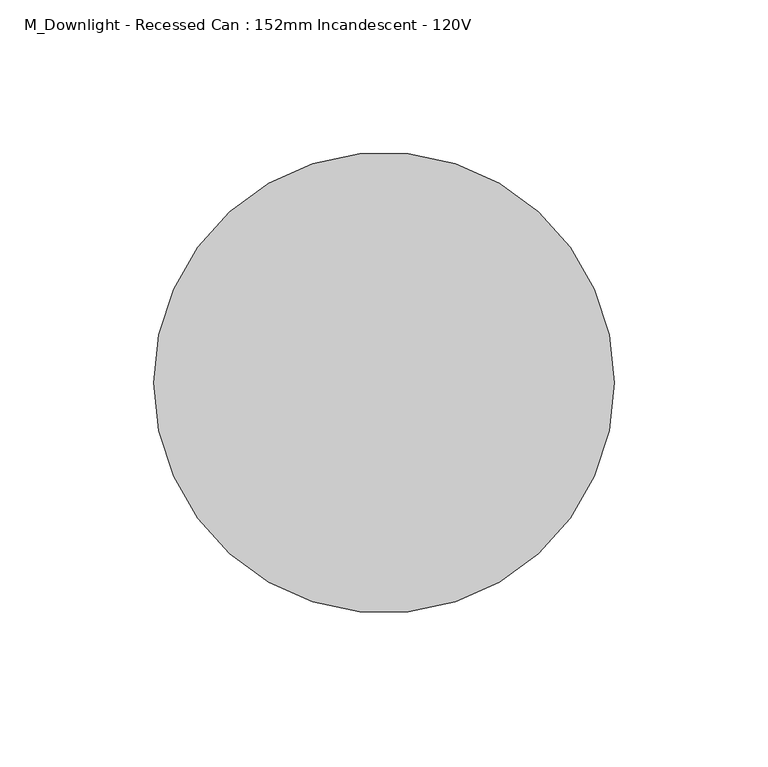
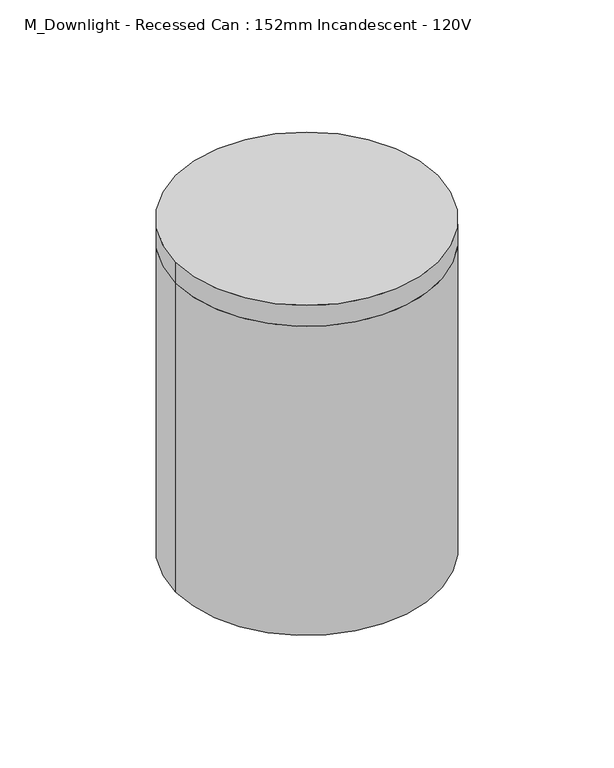
"""IFC4 building model written with IfcOpenShell, lengths in millimetres: light fixture geometry, M_Downlight - Recessed Can : 152mm Incandescent - 120V."""

from ifc_helpers import new_model, si_unit, point, frame, origin, origin_2d, place, context, project, spatial, circle_curve, trimmed, segment, composite_curve, outline, extrude, source, transform, mapped, element, save


def m_downlight_recessed_can_152mm_incandescent_120v_9e946963(model_context):
    return source(origin(), model_context, "Body", "SweptSolid", [
        extrude(outline(composite_curve([segment(trimmed(circle_curve(origin_2d(), 75.0), [point((-75.0, 0.0))], [point((75.0, 0.0))], False, "CARTESIAN"), True, "CONTINUOUS"), segment(trimmed(circle_curve(origin_2d(), 75.0), [point((75.0, 0.0))], [point((-75.0, 0.0))], False, "CARTESIAN"), True, "CONTINUOUS")], self_intersect=False)), frame((0.0, 0.0, 2625.7), z_axis=(0.0, 0.0, 1.0), x_axis=(1.0, 0.0, 0.0)), (0.0, 0.0, 1.0), 12.7),
        extrude(outline(composite_curve([segment(trimmed(circle_curve(origin_2d(), 75.0), [point((-75.0, 0.0))], [point((75.0, 0.0))], False, "CARTESIAN"), True, "CONTINUOUS"), segment(trimmed(circle_curve(origin_2d(), 75.0), [point((75.0, 0.0))], [point((-75.0, 0.0))], False, "CARTESIAN"), True, "CONTINUOUS")], self_intersect=False), holes=[composite_curve([segment(trimmed(circle_curve(origin_2d(), 62.3), [point((-62.3, 0.0))], [point((62.3, 0.0))], True, "CARTESIAN"), True, "CONTINUOUS"), segment(trimmed(circle_curve(origin_2d(), 62.3), [point((62.3, 0.0))], [point((-62.3, 0.0))], True, "CARTESIAN"), True, "CONTINUOUS")], self_intersect=False)]), frame((0.0, 0.0, 2438.4), z_axis=(0.0, 0.0, 1.0), x_axis=(1.0, 0.0, 0.0)), (0.0, 0.0, 1.0), 187.3),
    ])


if __name__ == "__main__":
    model = new_model("IFC4")
    model_context = context("Model", 3, world=origin())
    ifc_project = project(units=[si_unit("LENGTHUNIT", "METRE", prefix="MILLI")], contexts=[model_context])
    site = spatial("IfcSite", under=ifc_project)
    building = spatial("IfcBuilding", under=site)
    placement = place(None, origin())
    m_downlight_recessed_can_152mm_incandescent_120v_shape = m_downlight_recessed_can_152mm_incandescent_120v_9e946963(model_context)
    element("IfcLightFixture", 1, ObjectType="M_Downlight - Recessed Can : 152mm Incandescent - 120V", at=placement, inside=building, context=model_context, shape_type="MappedRepresentation", body=[
        mapped(m_downlight_recessed_can_152mm_incandescent_120v_shape, transform((0.0, 0.0, 0.0), x_axis=(1.0, 0.0, 0.0), y_axis=(0.0, 1.0, 0.0), z_axis=(0.0, 0.0, 1.0))),
    ])
    save(model, "model.ifc")

# Revit data of these elements
# Type "M_Downlight - Recessed Can : 152mm Incandescent - 120V"
#   Assembly Code = "D5020220"
#   Lamp = "A-19"
#   Wattage = 60 W
#   built-in parameter 1150110 = 1 (stored number, unit not read)
#   built-in parameter 1114217 = 1 (stored number, unit not read)
#   built-in parameter 1150109 = 1 (stored number, unit not read)
#   built-in parameter 1150113 = 1 (stored number, unit not read)
#   Tilt Angle = 90.00°
#   built-in parameter 1010507 = 1.5708 (stored number, unit not read)
#   built-in parameter 1010506 = 0.523599 (stored number, unit not read)
#   Recessing Radius = 75 mm
#   Recessing Inner Radius = 62.3 mm
#   built-in parameter 1150115 = 1 (stored number, unit not read)
#   built-in parameter 1150105 = 2858.75 (stored number, unit not read)
#   Light Source Symbol Length = 3048 mm
#   built-in parameter 1150112 = 1 (stored number, unit not read)
#   built-in parameter 1150114 = 1 (stored number, unit not read)
#   built-in parameter 1150107 = 2800 (stored number, unit not read)
#   built-in parameter 1150106 = 28.5875 (stored number, unit not read)
#   built-in parameter 1150104 = 1.32387 (stored number, unit not read)
#   Ballast Voltage = 120 V
#   built-in parameter 1114218 = 1 (stored number, unit not read)
#   built-in parameter 1150133 = 10 (stored number, unit not read)
#   Recessing Height = 200 mm
#   Recessing Diameter = 150 mm
#   Lumens = 855 lm
#   Apparent Load = 60 VA
#   built-in parameter 1150134 = 4
#   built-in parameter 1150137 = 1
#   Color Filter = 16777215
#   Ballast Number of Poles = 1
#   Material = none
#   Load Classification = Lighting - Dwelling Unit
#   Dimming Lamp Color Temperature Shift = (empty or 0)
#   Default Elevation = 0
#   Wattage Comments = ""
